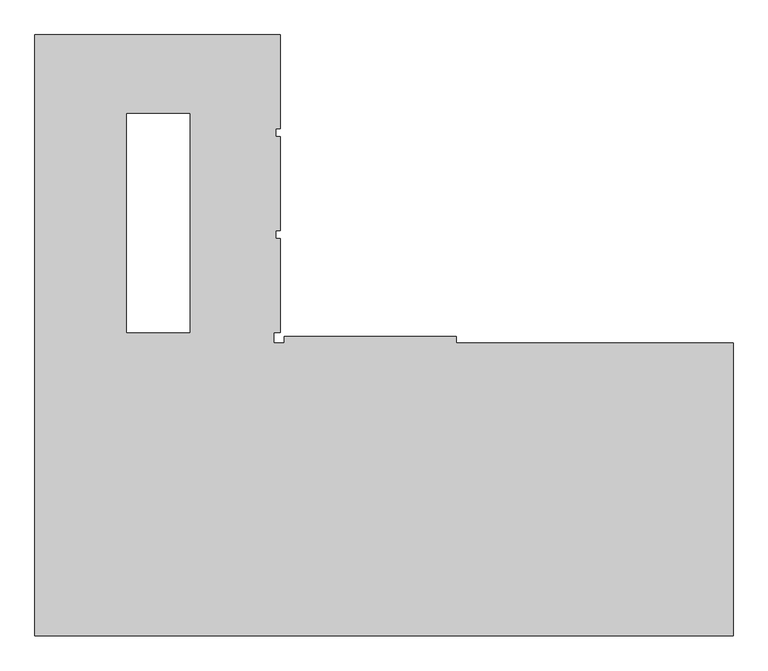
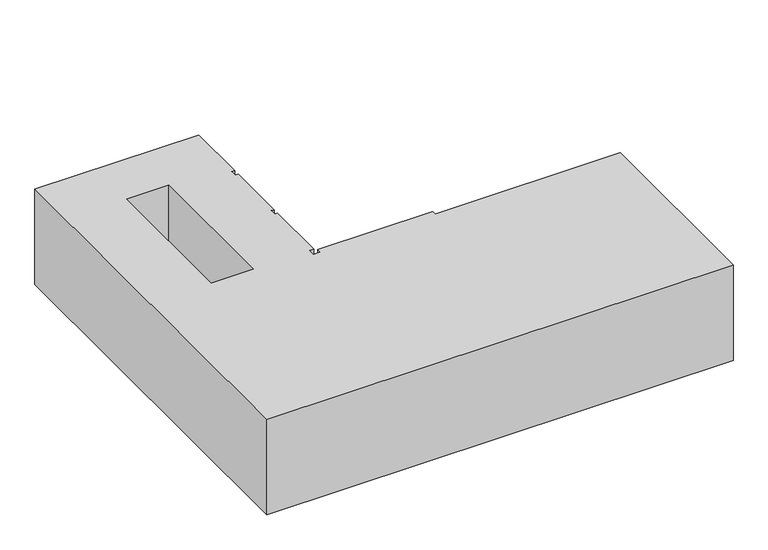
"""IFC4 building model written with IfcOpenShell, lengths in millimetres: proxy geometry, 0_3d."""

import ifcopenshell
import ifcopenshell.guid

model = None  # the IFC model being written
_history = None  # IfcOwnerHistory: only IFC2X3 demands one
_inside = {}  # id of a spatial element -> (the spatial element, [elements in it])
_under = {}  # id of a project, library or spatial element -> (it, [spatial elements below it])
_declared = {}  # id of a project -> (the project, [libraries it declares])
_typed = {}  # id of a type object -> (the type object, [elements of that type])
_made_of = {}  # id of a material, layer set ... -> (it, [elements and type objects made of it])


def new_model(schema):
    """Start an empty IFC model of exactly this schema.

    Asked for "IFC4X3", IfcOpenShell would pick the latest addendum, in which some entities
    have other attributes; the version numbers below select the first issue.
    IFC2X3 requires an IfcOwnerHistory on every rooted entity: one is made here for all.
    """
    global model, _history
    if schema == "IFC4X3":
        model = ifcopenshell.file(schema_version=(4, 3, 0, 0))
    else:
        model = ifcopenshell.file(schema=schema)
    _inside.clear()
    _under.clear()
    _declared.clear()
    _typed.clear()
    _made_of.clear()
    _history = None
    if model.schema == "IFC2X3":
        org = make("IfcOrganization", Name="unknown")
        user = make(
            "IfcPersonAndOrganization",
            ThePerson=make("IfcPerson", FamilyName="unknown"),
            TheOrganization=org,
        )
        app = make(
            "IfcApplication",
            ApplicationDeveloper=org,
            Version="unknown",
            ApplicationFullName="unknown",
            ApplicationIdentifier="unknown",
        )
        _history = make(
            "IfcOwnerHistory",
            OwningUser=user,
            OwningApplication=app,
            ChangeAction="ADDED",
            CreationDate=0,
        )
    return model


def make(cls, **values):
    """One entity of the class cls with the attributes given. An attribute that is None is left unset."""
    return model.create_entity(
        cls, **{name: value for name, value in values.items() if value is not None}
    )


def rooted(cls, **values):
    """An entity with a GlobalId (a new one), such as an element, a storey or a relation."""
    return make(cls, GlobalId=ifcopenshell.guid.new(), OwnerHistory=_history, **values)


def si_unit(unit_type, name, prefix=None):
    """IfcSIUnit, for example si_unit("LENGTHUNIT", "METRE", prefix="MILLI")."""
    return make("IfcSIUnit", UnitType=unit_type, Prefix=prefix, Name=name)


def assignment(units):
    """IfcUnitAssignment: the units of a project."""
    return None if units is None else make("IfcUnitAssignment", Units=units)


def point(xyz):
    """IfcCartesianPoint."""
    return None if xyz is None else make("IfcCartesianPoint", Coordinates=xyz)


def direction(xyz):
    """IfcDirection."""
    return None if xyz is None else make("IfcDirection", DirectionRatios=xyz)


def frame(location, z_axis=None, x_axis=None):
    """IfcAxis2Placement3D, a coordinate frame: its origin and axes. An axis left out is left unset."""
    return make(
        "IfcAxis2Placement3D",
        Location=point(location),
        Axis=direction(z_axis),
        RefDirection=direction(x_axis),
    )


def origin():
    """The frame at (0, 0, 0) with its axes left unset."""
    return frame((0.0, 0.0, 0.0))


def origin_with_axes():
    """The frame at (0, 0, 0) with the z axis (0, 0, 1) and the x axis (1, 0, 0) written out."""
    return frame((0.0, 0.0, 0.0), z_axis=(0.0, 0.0, 1.0), x_axis=(1.0, 0.0, 0.0))


def place(relative_to, where):
    """IfcLocalPlacement: puts the frame where relative to a parent placement (None: the world)."""
    return make(
        "IfcLocalPlacement", PlacementRelTo=relative_to, RelativePlacement=where
    )


def context(
    kind, dimensions, precision=None, world=None, true_north=None, identifier=None
):
    """IfcGeometricRepresentationContext, for example the 3D "Model" context."""
    return make(
        "IfcGeometricRepresentationContext",
        ContextIdentifier=identifier,
        ContextType=kind,
        CoordinateSpaceDimension=dimensions,
        Precision=precision,
        WorldCoordinateSystem=world,
        TrueNorth=true_north,
    )


def project(units=None, contexts=None):
    """IfcProject with its units and contexts."""
    return rooted(
        "IfcProject",
        Name="project",
        RepresentationContexts=contexts,
        UnitsInContext=assignment(units),
    )


def spatial(cls, under=None, at=None, **own):
    """A site, building, storey or space (cls), placed at a placement, below another one or the project."""
    s = rooted(cls, ObjectPlacement=at, **own)
    if under is not None:
        _under.setdefault(under.id(), (under, []))[1].append(s)
    return s


def polyline(points):
    """IfcPolyline through the points."""
    return make("IfcPolyline", Points=[point(p) for p in points])


def outline(outer, holes=None, kind="AREA"):
    """IfcArbitraryClosedProfileDef: a profile drawn as a closed curve; with holes, ...WithVoids."""
    if holes is None:
        return make("IfcArbitraryClosedProfileDef", ProfileType=kind, OuterCurve=outer)
    return make(
        "IfcArbitraryProfileDefWithVoids",
        ProfileType=kind,
        OuterCurve=outer,
        InnerCurves=holes,
    )


def extrude(swept, where, along, depth):
    """IfcExtrudedAreaSolid: the profile swept, set in the frame where, extruded along a direction by depth."""
    return make(
        "IfcExtrudedAreaSolid",
        SweptArea=swept,
        Position=where,
        ExtrudedDirection=direction(along),
        Depth=depth,
    )


def shape(context_of_items, identifier, shape_type, items):
    """IfcShapeRepresentation: the items that make up one representation, for example the "Body"."""
    return make(
        "IfcShapeRepresentation",
        ContextOfItems=context_of_items,
        RepresentationIdentifier=identifier,
        RepresentationType=shape_type,
        Items=items,
    )


def source(mapping_origin, context_of_items, identifier, shape_type, items):
    """IfcRepresentationMap: a shape defined once, which mapped items show again and again."""
    return make(
        "IfcRepresentationMap",
        MappingOrigin=mapping_origin,
        MappedRepresentation=shape(context_of_items, identifier, shape_type, items),
    )


def transform(
    local_origin,
    x_axis=None,
    y_axis=None,
    z_axis=None,
    scale=None,
    scale2=None,
    scale3=None,
    uniform=True,
):
    """IfcCartesianTransformationOperator3D, or its non-uniform kind. x_axis, y_axis, z_axis: its Axis1, 2, 3."""
    if uniform:
        return make(
            "IfcCartesianTransformationOperator3D",
            Axis1=direction(x_axis),
            Axis2=direction(y_axis),
            LocalOrigin=point(local_origin),
            Scale=scale,
            Axis3=direction(z_axis),
        )
    return make(
        "IfcCartesianTransformationOperator3DnonUniform",
        Axis1=direction(x_axis),
        Axis2=direction(y_axis),
        LocalOrigin=point(local_origin),
        Scale=scale,
        Axis3=direction(z_axis),
        Scale2=scale2,
        Scale3=scale3,
    )


def mapped(mapping_source, mapping_target):
    """IfcMappedItem: shows the shape of a source again, moved by a transform."""
    return make(
        "IfcMappedItem", MappingSource=mapping_source, MappingTarget=mapping_target
    )


def made_of(thing, what):
    """Note that an element or type object is made of a material, layer set ...; save() writes the relation."""
    if what is not None:
        _made_of.setdefault(what.id(), (what, []))[1].append(thing)
    return thing


def element(
    cls,
    number,
    at=None,
    inside=None,
    cuts=None,
    type_object=None,
    material=None,
    context=None,
    identifier="Body",
    shape_type=None,
    held_by="IfcProductDefinitionShape",
    body=None,
    shapes=None,
    **own,
):
    """One element of the class cls, such as IfcWall. Its Tag is "e" and its number.

    at: its placement. inside: the storey or other place that contains it. cuts: it is an
    opening in that element (IfcRelVoidsElement). A single representation is given by context,
    identifier, shape_type and body (its items); several are given by shapes. held_by: the class
    of the entity that holds the representations. save() writes the other relations.
    """
    e = rooted(cls, Tag="e%d" % number, ObjectPlacement=at, **own)
    if body is not None:
        shapes = [shape(context, identifier, shape_type, body)]
    if shapes is not None:
        e.Representation = make(held_by, Representations=shapes)
    if inside is not None:
        _inside.setdefault(inside.id(), (inside, []))[1].append(e)
    if cuts is not None:
        rooted(
            "IfcRelVoidsElement", RelatingBuildingElement=cuts, RelatedOpeningElement=e
        )
    if type_object is not None:
        _typed.setdefault(type_object.id(), (type_object, []))[1].append(e)
    return made_of(e, material)


def aggregate(whole, parts):
    """IfcRelAggregates: a whole, such as a stair, and the parts it consists of."""
    return rooted("IfcRelAggregates", RelatingObject=whole, RelatedObjects=parts)


def save(model, path):
    """Write the relations noted so far, then the file.

    IfcRelAggregates (storeys below a building ...), IfcRelContainedInSpatialStructure (elements
    in a storey), IfcRelDefinesByType, IfcRelAssociatesMaterial and IfcRelDeclares: one each for
    every whole, place, type object, material and project.
    """
    for whole, parts in _under.values():
        aggregate(whole, parts)
    for where, things in _inside.values():
        rooted(
            "IfcRelContainedInSpatialStructure",
            RelatedElements=things,
            RelatingStructure=where,
        )
    for kind, things in _typed.values():
        rooted("IfcRelDefinesByType", RelatedObjects=things, RelatingType=kind)
    for what, things in _made_of.values():
        rooted("IfcRelAssociatesMaterial", RelatedObjects=things, RelatingMaterial=what)
    for by, libraries in _declared.values():
        rooted("IfcRelDeclares", RelatingContext=by, RelatedDefinitions=libraries)
    model.write(path)


def generic_models_b5a4028e(model_context):
    return source(origin(), model_context, "Body", "SweptSolid", [
        extrude(outline(polyline([(4550.0, 5582.8619019), (4750.0, 5582.8619019), (4750.0, 5704.8619019), (8028.0, 5704.8619019), (8028.0, 5582.8619019), (13300.0, 5582.8619019), (13300.0, 0.0), (0.0, 0.0), (0.0, 11452.8619019), (4672.0, 11452.8619019), (4672.0, 9669.4619019), (4590.0, 9669.4619019), (4590.0, 9509.4619019), (4672.0, 9509.4619019), (4672.0, 7726.1619019), (4590.0, 7726.1619019), (4590.0, 7566.1619019), (4672.0, 7566.1619019), (4672.0, 5782.8619019), (4550.0, 5782.8619019), (4550.0, 5582.8619019)]), holes=[polyline([(2949.4613155, 5782.8619019), (2949.4613155, 9952.8619019), (1748.7090817, 9952.8619019), (1748.7090817, 5782.8619019), (2949.4613155, 5782.8619019)])]), origin_with_axes(), (0.0, 0.0, 1.0), 2880.0),
    ])


if __name__ == "__main__":
    model = new_model("IFC4")
    model_context = context("Model", 3, world=origin())
    ifc_project = project(units=[si_unit("LENGTHUNIT", "METRE", prefix="MILLI")], contexts=[model_context])
    site = spatial("IfcSite", under=ifc_project)
    building = spatial("IfcBuilding", under=site)
    placement = place(None, origin())
    generic_models_shape = generic_models_b5a4028e(model_context)
    element("IfcBuildingElementProxy", 1, Name="0_3d", ObjectType="0_3d", at=placement, inside=building, context=model_context, shape_type="MappedRepresentation", body=[
        mapped(generic_models_shape, transform((0.0, 0.0, 0.0), x_axis=(1.0, 0.0, 0.0), y_axis=(0.0, 1.0, 0.0), z_axis=(0.0, 0.0, 1.0))),
    ])
    save(model, "model.ifc")

# Revit data of these elements
# Element 1 (IfcBuildingElementProxy, "0_3d")
#   Materials on its faces: "*1"
# Materials
#   "*1": class "Unassigned", colour RGB 175 175 175, transparency 0
